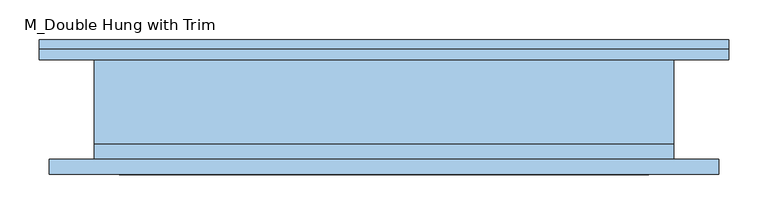
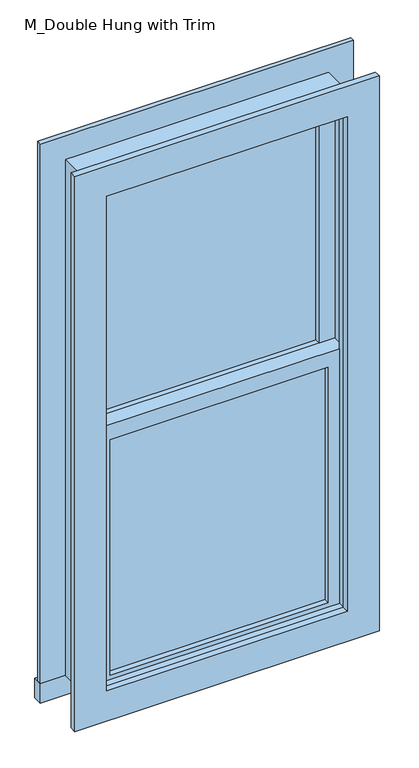
"""IFC4 building model written with IfcOpenShell, lengths in millimetres: window geometry, M_Double Hung with Trim."""

from ifc_helpers import new_model, si_unit, frame, origin, place, context, project, spatial, polyline, outline, extrude, source, transform, mapped, element, save


def m_double_hung_with_trim_52fe8b26(model_context):
    return source(origin(), model_context, "Body", "SweptSolid", [
        extrude(outline(polyline([(-304.8, -15.825), (304.8, -15.825), (304.8, -28.525), (-304.8, -28.525), (-304.8, -15.825)])), frame((0.0, 0.0, 628.65), z_axis=(0.0, 0.0, 1.0), x_axis=(1.0, 0.0, 0.0)), (0.0, 0.0, 1.0), 695.325),
        extrude(outline(polyline([(1368.425, -349.25), (584.2, -349.25), (584.2, 349.25), (1368.425, 349.25), (1368.425, -349.25)]), holes=[polyline([(1323.975, -304.8), (1323.975, 304.8), (628.65, 304.8), (628.65, -304.8), (1323.975, -304.8)])]), frame((0.0, -44.4, 0.0), z_axis=(0.0, 1.0, 0.0), x_axis=(0.0, 0.0, 1.0)), (0.0, 0.0, 1.0), 44.45),
        extrude(outline(polyline([(-438.25, 89.2), (438.25, 89.2), (438.25, 63.5), (-438.25, 63.5), (-438.25, 89.2)])), frame((0.0, 0.0, 526.95), z_axis=(0.0, 0.0, 1.0), x_axis=(1.0, 0.0, 0.0)), (0.0, 0.0, 1.0), 57.25),
        extrude(outline(polyline([(2178.15, -438.25), (526.95, -438.25), (526.95, 438.25), (2178.15, 438.25), (2178.15, -438.25)]), holes=[polyline([(2089.15, -349.25), (2089.15, 349.25), (584.2, 349.25), (584.2, -349.25), (2089.15, -349.25)])]), frame((0.0, 63.5, 0.0), z_axis=(0.0, 1.0, 0.0), x_axis=(0.0, 0.0, 1.0)), (0.0, 0.0, 1.0), 13.0),
        extrude(outline(polyline([(2165.45, 425.55), (2165.45, -425.55), (526.95, -425.55), (526.95, 425.55), (2165.45, 425.55)]), holes=[polyline([(2076.45, 336.55), (615.95, 336.55), (615.95, -336.55), (2076.45, -336.55), (2076.45, 336.55)])]), frame((0.0, -82.5, 0.0), z_axis=(0.0, 1.0, 0.0), x_axis=(0.0, 0.0, 1.0)), (0.0, 0.0, 1.0), 19.0),
        extrude(outline(polyline([(304.8, 15.925), (-304.8, 15.925), (-304.8, 28.625), (304.8, 28.625), (304.8, 15.925)])), frame((0.0, 0.0, 1368.425), z_axis=(0.0, 0.0, 1.0), x_axis=(1.0, 0.0, 0.0)), (0.0, 0.0, 1.0), 676.275),
        extrude(outline(polyline([(2089.15, -349.25), (1323.975, -349.25), (1323.975, 349.25), (2089.15, 349.25), (2089.15, -349.25)]), holes=[polyline([(2044.7, -304.8), (2044.7, 304.8), (1368.425, 304.8), (1368.425, -304.8), (2044.7, -304.8)])]), frame((0.0, 0.05, 0.0), z_axis=(0.0, 1.0, 0.0), x_axis=(0.0, 0.0, 1.0)), (0.0, 0.0, 1.0), 44.45),
        extrude(outline(polyline([(2108.2, -368.3), (584.2, -368.3), (584.2, 368.3), (2108.2, 368.3), (2108.2, -368.3)]), holes=[polyline([(2076.45, -336.55), (2076.45, 336.55), (615.95, 336.55), (615.95, -336.55), (2076.45, -336.55)])]), frame((0.0, -63.5, 0.0), z_axis=(0.0, 1.0, 0.0), x_axis=(0.0, 0.0, 1.0)), (0.0, 0.0, 1.0), 19.1),
        extrude(outline(polyline([(2108.2, 368.3), (2108.2, -368.3), (584.2, -368.3), (584.2, 368.3), (2108.2, 368.3)]), holes=[polyline([(2089.15, 349.25), (603.25, 349.25), (603.25, -349.25), (2089.15, -349.25), (2089.15, 349.25)])]), frame((0.0, -44.4, 0.0), z_axis=(0.0, 1.0, 0.0), x_axis=(0.0, 0.0, 1.0)), (0.0, 0.0, 1.0), 107.9),
    ])


if __name__ == "__main__":
    model = new_model("IFC4")
    model_context = context("Model", 3, world=origin())
    ifc_project = project(units=[si_unit("LENGTHUNIT", "METRE", prefix="MILLI")], contexts=[model_context])
    site = spatial("IfcSite", under=ifc_project)
    building = spatial("IfcBuilding", under=site)
    placement = place(None, origin())
    m_double_hung_with_trim_shape = m_double_hung_with_trim_52fe8b26(model_context)
    element("IfcWindow", 1, ObjectType="M_Double Hung with Trim : 29\" x 60\" @ 23\"", at=placement, inside=building, context=model_context, shape_type="MappedRepresentation", body=[
        mapped(m_double_hung_with_trim_shape, transform((0.0, 0.0, 0.0), x_axis=(1.0, 0.0, 0.0), y_axis=(0.0, 1.0, 0.0), z_axis=(0.0, 0.0, 1.0))),
    ])
    save(model, "model.ifc")

# Revit data of these elements
# Type "M_Double Hung with Trim : 29\" x 60\" @ 23\""
#   Type Mark = "61"
#   Construction Type Id = "GSP4R"
#   Analytic Construction = "1/8 in Pilkington single glazing"
#   Visual Light Transmittance = 0.9
#   Thermal Resistance (R) = 0.271106 (m²·K)/W
#   Solar Heat Gain Coefficient = 0.78
#   Heat Transfer Coefficient (U) = 3.6886 W/(m²·K)
#   Height = 5' - 0"
#   Default Sill Height = 1' - 11"
#   Trim Projection - Ext. = 0' - 0.51181"
#   Trim Projection - Int. = 0' - 0.74803"
#   Trim Width - Exterior = 0' - 3.50394"
#   Trim Width - Interior = 0' - 3.50394"
#   Width = 2' - 5"
#   Window Inset = 0' - 0.74803"
#   Glass Pane Material = EXISTING WINDOW
#   Sash = Trim
#   Trim Exterior Material = Trim
#   Trim Interior Material = Trim
#   Wall Closure = (empty or 0)
# Element 1 (IfcWindow, "M_Double Hung with Trim : 29\" x 60\" @ 23\"")
#   Materials on its faces: "Trim", "EXISTING WINDOW"
# Materials
#   "EXISTING WINDOW": class "Glass", colour RGB 218 227 224, transparency 0.85, Description = "Soda Lime Glass", Cost = 0
#   "Trim": class "Wood", colour RGB 250 251 245, transparency 0, Cost = 0
